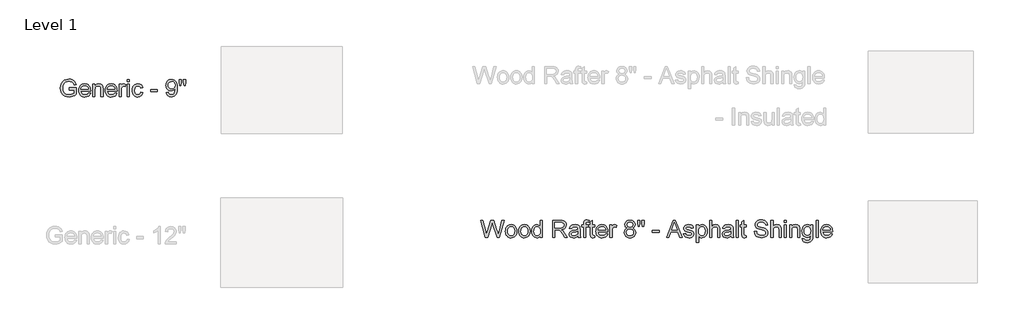
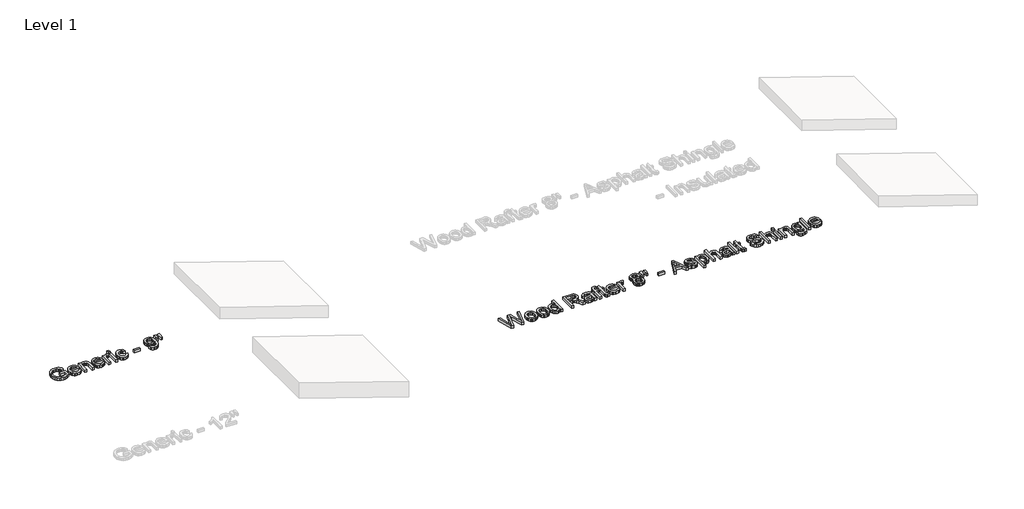
# One storey, part 7 of 42: 2 proxies.
"""IFC4 building model written with IfcOpenShell, lengths in millimetres."""

from ifc_helpers import new_model, si_unit, origin, origin_with_axes, place, context, project, spatial, polyline, outline, extrude, element, save

model = new_model("IFC4")

# Units and contexts
model_context = context("Model", 3, world=origin())
ifc_project = project(units=[si_unit("LENGTHUNIT", "METRE", prefix="MILLI")], contexts=[model_context])

# Site, building, storey
site = spatial("IfcSite", under=ifc_project)
building = spatial("IfcBuilding", under=site)
storey = spatial("IfcBuildingStorey", under=building, Name="Level 1", Elevation=0.0)

# Proxies
placement = place(None, origin())
element("IfcBuildingElementProxy", 1, Name="8\" Arial", ObjectType="8\" Arial", at=placement, inside=storey, context=model_context, shape_type="SweptSolid", body=[
    extrude(outline(polyline([(-15459.1576227, -5830.4947741), (-15459.1576227, -5792.4238873), (-15335.4272408, -5792.4238873), (-15335.4272408, -5906.2647616), (-15365.4954338, -5927.1777243), (-15396.5116812, -5942.1792895), (-15428.4016256, -5951.2136894), (-15461.09091, -5954.2251561), (-15503.7998271, -5949.4384113), (-15542.4005089, -5935.0781769), (-15574.4670517, -5911.646364), (-15597.5735518, -5879.6448838), (-15611.5434109, -5841.2579789), (-15616.2000306, -5798.6698922), (-15611.5620002, -5755.775082), (-15597.647909, -5715.8731492), (-15575.0340254, -5682.4031143), (-15560.680762, -5669.3696912), (-15544.2966175, -5658.8039977), (-15506.857767, -5644.8062546), (-15464.1395552, -5640.1403403), (-15432.7794058, -5642.8450835), (-15404.5794374, -5650.959313), (-15380.8316065, -5663.8974659), (-15362.8278692, -5681.0739793), (-15349.5086357, -5703.3160769), (-15339.8143156, -5731.4509828), (-15374.9109143, -5741.3404905), (-15382.7463044, -5721.2733409), (-15392.2733207, -5706.1323559), (-15404.8768662, -5694.7185256), (-15421.9418438, -5685.8328401), (-15442.2878328, -5680.1166303), (-15464.7344128, -5678.2112271), (-15491.0103886, -5680.2653447), (-15513.4755579, -5686.4276977), (-15532.0462687, -5695.9268301), (-15546.6388694, -5707.9912859), (-15566.2319917, -5737.3252016), (-15575.1548558, -5766.0642597), (-15578.1291439, -5797.108391), (-15574.5507036, -5833.5155354), (-15563.8153827, -5863.4721926), (-15546.2484941, -5886.7645857), (-15522.1753503, -5903.1789378), (-15494.0032659, -5912.9104364), (-15464.1395552, -5916.1542693), (-15437.7706329, -5913.7097763), (-15412.0523361, -5906.3762974), (-15389.7172919, -5896.2730128), (-15373.4981275, -5885.5191026), (-15373.4981275, -5830.4947741), (-15459.1576227, -5830.4947741)])), origin_with_axes(), (0.0, 0.0, 1.0), 50.8),
    extrude(outline(polyline([(-15121.724646, -5882.8422434), (-15084.3973312, -5887.6011042), (-15097.8466899, -5915.7267154), (-15119.3080369, -5936.7512139), (-15148.2980506, -5949.8566705), (-15184.333409, -5954.2251561), (-15207.9557621, -5952.3406658), (-15229.0034973, -5946.6871948), (-15247.4766143, -5937.2647433), (-15263.3751133, -5924.0733112), (-15276.1599045, -5907.4800371), (-15285.2918982, -5887.8520598), (-15290.7710944, -5865.1893792), (-15292.5974932, -5839.4919954), (-15290.7525051, -5812.9232381), (-15285.217541, -5789.5053672), (-15275.9926008, -5769.2383827), (-15263.0776845, -5752.1222846), (-15247.2210114, -5738.5242115), (-15229.170801, -5728.8113021), (-15208.9270531, -5722.9835565), (-15186.4897678, -5721.0409747), (-15164.7751415, -5722.9789092), (-15145.1378695, -5728.7927128), (-15127.5779519, -5738.4823856), (-15112.0953885, -5752.0479274), (-15099.456988, -5769.1268469), (-15090.4295591, -5789.3566528), (-15085.0131018, -5812.7373451), (-15083.207616, -5839.2689238), (-15083.4306876, -5849.5302175), (-15254.5266064, -5849.5302175), (-15247.9366995, -5878.0276146), (-15232.6284108, -5898.9777559), (-15210.5350275, -5911.860141), (-15183.5898369, -5916.1542693), (-15163.3274998, -5914.1652142), (-15146.2625222, -5908.1980488), (-15132.3949043, -5897.8809872), (-15121.724646, -5882.8422434)]), holes=[polyline([(-15254.5266064, -5811.4593307), (-15121.2785028, -5811.4593307), (-15126.4277389, -5791.3457079), (-15136.5217289, -5776.9575896), (-15158.7173533, -5763.5732935), (-15186.6384822, -5759.1118614), (-15212.3010111, -5762.6717124), (-15233.5206972, -5773.3512654), (-15248.2713069, -5789.9979837), (-15254.5266064, -5811.4593307)])]), origin_with_axes(), (0.0, 0.0, 1.0), 50.8),
    extrude(outline(polyline([(-15045.1367292, -5949.4662952), (-15045.1367292, -5725.7998355), (-15007.0658425, -5725.7998355), (-15007.0658425, -5757.0298598), (-14993.8395554, -5741.2847226), (-14977.9549984, -5730.0381959), (-14959.4121715, -5723.29028), (-14938.2110746, -5721.0409747), (-14919.4451761, -5722.8534314), (-14902.2593681, -5728.2908017), (-14887.9270177, -5736.6745761), (-14877.7214919, -5747.3262451), (-14866.3076616, -5775.3217312), (-14864.3000171, -5812.1285455), (-14864.3000171, -5949.4662952), (-14902.3709039, -5949.4662952), (-14902.3709039, -5817.2591924), (-14906.7579787, -5783.5753805), (-14912.8273852, -5773.546453), (-14922.2614551, -5765.7668309), (-14934.3537948, -5760.7756038), (-14948.3980111, -5759.1118614), (-14970.6958767, -5762.8483108), (-14989.7034361, -5774.0576588), (-14997.2994889, -5783.2082418), (-15002.7252409, -5795.7141935), (-15007.0658425, -5830.7922029), (-15007.0658425, -5949.4662952), (-15045.1367292, -5949.4662952)])), origin_with_axes(), (0.0, 0.0, 1.0), 50.8),
    extrude(outline(polyline([(-14655.3562832, -5882.8422434), (-14618.0289684, -5887.6011042), (-14631.4783271, -5915.7267154), (-14652.9396741, -5936.7512139), (-14681.9296878, -5949.8566705), (-14717.9650462, -5954.2251561), (-14741.5873994, -5952.3406658), (-14762.6351345, -5946.6871948), (-14781.1082515, -5937.2647433), (-14797.0067505, -5924.0733112), (-14809.7915417, -5907.4800371), (-14818.9235354, -5887.8520598), (-14824.4027316, -5865.1893792), (-14826.2291304, -5839.4919954), (-14824.3841423, -5812.9232381), (-14818.8491782, -5789.5053672), (-14809.624238, -5769.2383827), (-14796.7093217, -5752.1222846), (-14780.8526487, -5738.5242115), (-14762.8024382, -5728.8113021), (-14742.5586903, -5722.9835565), (-14720.121405, -5721.0409747), (-14698.4067787, -5722.9789092), (-14678.7695067, -5728.7927128), (-14661.2095891, -5738.4823856), (-14645.7270257, -5752.0479274), (-14633.0886252, -5769.1268469), (-14624.0611963, -5789.3566528), (-14618.644739, -5812.7373451), (-14616.8392532, -5839.2689238), (-14617.0623248, -5849.5302175), (-14788.1582436, -5849.5302175), (-14781.5683367, -5878.0276146), (-14766.260048, -5898.9777559), (-14744.1666648, -5911.860141), (-14717.2214742, -5916.1542693), (-14696.959137, -5914.1652142), (-14679.8941594, -5908.1980488), (-14666.0265415, -5897.8809872), (-14655.3562832, -5882.8422434)]), holes=[polyline([(-14788.1582436, -5811.4593307), (-14654.91014, -5811.4593307), (-14660.0593761, -5791.3457079), (-14670.1533661, -5776.9575896), (-14692.3489905, -5763.5732935), (-14720.2701194, -5759.1118614), (-14745.9326483, -5762.6717124), (-14767.1523344, -5773.3512654), (-14781.9029441, -5789.9979837), (-14788.1582436, -5811.4593307)])]), origin_with_axes(), (0.0, 0.0, 1.0), 50.8),
    extrude(outline(polyline([(-14578.7683664, -5949.4662952), (-14578.7683664, -5725.7998355), (-14545.4563405, -5725.7998355), (-14545.4563405, -5758.8887898), (-14533.1502238, -5739.704632), (-14521.8107507, -5728.4023375), (-14510.434099, -5722.8813154), (-14498.0164465, -5721.0409747), (-14479.0553603, -5723.9780841), (-14459.7968453, -5732.7894124), (-14472.5119266, -5766.9193675), (-14485.8962228, -5761.0637379), (-14499.2805189, -5759.1118614), (-14510.647876, -5760.9893807), (-14520.8069285, -5766.6219387), (-14529.0141045, -5775.5819814), (-14534.525832, -5787.4419549), (-14539.1545678, -5808.7081143), (-14540.6974797, -5831.9075609), (-14540.6974797, -5949.4662952), (-14578.7683664, -5949.4662952)])), origin_with_axes(), (0.0, 0.0, 1.0), 50.8),
    extrude(outline(polyline([(-14436.0025411, -5682.9700879), (-14436.0025411, -5644.8992011), (-14397.9316543, -5644.8992011), (-14397.9316543, -5682.9700879), (-14436.0025411, -5682.9700879)])), origin_with_axes(), (0.0, 0.0, 1.0), 50.8),
    extrude(outline(polyline([(-14436.0025411, -5949.4662952), (-14436.0025411, -5725.7998355), (-14397.9316543, -5725.7998355), (-14397.9316543, -5949.4662952), (-14436.0025411, -5949.4662952)])), origin_with_axes(), (0.0, 0.0, 1.0), 50.8),
    extrude(outline(polyline([(-14198.0594989, -5868.5656609), (-14159.9886121, -5873.3245217), (-14170.6031025, -5907.184932), (-14190.5494216, -5932.7731037), (-14217.9500501, -5948.862143), (-14250.9274686, -5954.2251561), (-14272.2796035, -5952.3546077), (-14291.424259, -5946.7429627), (-14308.3614351, -5937.3902211), (-14323.0911318, -5924.2963828), (-14335.0138442, -5907.707756), (-14343.5300674, -5887.8706491), (-14348.6398013, -5864.7850619), (-14350.3430459, -5838.4509946), (-14347.4338204, -5804.571995), (-14338.706144, -5775.2101954), (-14324.0205969, -5751.499543), (-14303.2377593, -5734.5739852), (-14278.3745703, -5724.4242273), (-14251.447969, -5721.0409747), (-14219.279185, -5725.6882997), (-14193.5608882, -5739.6302748), (-14175.1110078, -5762.1233281), (-14164.747473, -5792.4238873), (-14202.8183597, -5797.1827482), (-14209.7242847, -5780.5732085), (-14220.4781949, -5768.6667617), (-14234.4852326, -5761.5005865), (-14251.1505402, -5759.1118614), (-14275.7534789, -5763.8149544), (-14295.2815388, -5777.9242332), (-14308.024504, -5802.2018592), (-14312.2721591, -5837.4099938), (-14308.1174506, -5873.0921554), (-14295.6533248, -5897.4534333), (-14276.4784617, -5911.4790603), (-14252.191541, -5916.1542693), (-14232.4775881, -5913.2357492), (-14216.3141916, -5904.4801888), (-14204.5564593, -5889.6645166), (-14198.0594989, -5868.5656609)])), origin_with_axes(), (0.0, 0.0, 1.0), 50.8),
    extrude(outline(polyline([(-14026.7405085, -5859.0479392), (-14026.7405085, -5820.9770524), (-13907.7689873, -5820.9770524), (-13907.7689873, -5859.0479392), (-14026.7405085, -5859.0479392)])), origin_with_axes(), (0.0, 0.0, 1.0), 50.8),
    extrude(outline(polyline([(-13750.7265795, -5873.3245217), (-13712.6556927, -5868.5656609), (-13706.1494376, -5890.1757223), (-13695.5535365, -5904.8891534), (-13681.1282396, -5913.3379903), (-13663.133797, -5916.1542693), (-13646.9889898, -5914.3418125), (-13632.3127373, -5908.9044422), (-13620.1181564, -5900.437016), (-13611.4183639, -5889.5343915), (-13598.9635328, -5856.4454371), (-13593.4611, -5812.2772599), (-13593.6841716, -5804.8415399), (-13606.87328, -5820.9398738), (-13624.1334453, -5833.6921337), (-13644.2191841, -5842.0015509), (-13665.8850135, -5844.7713566), (-13683.9700789, -5843.0797303), (-13700.6005315, -5838.0048514), (-13715.7763715, -5829.5467198), (-13729.4975987, -5817.7053356), (-13740.8672794, -5803.098793), (-13748.9884799, -5786.3451862), (-13753.8612002, -5767.4445152), (-13755.4854403, -5746.3967801), (-13753.7821957, -5724.6472989), (-13748.6724618, -5705.1285337), (-13740.1562386, -5687.8404846), (-13728.2335262, -5672.7831514), (-13713.7454904, -5660.5839232), (-13697.533297, -5651.8701887), (-13679.596946, -5646.641948), (-13659.9364374, -5644.8992011), (-13631.5412814, -5648.8773114), (-13605.6928595, -5660.8116421), (-13584.0735034, -5680.1073357), (-13568.3655447, -5706.1695345), (-13558.8013498, -5742.1955983), (-13555.6132848, -5791.3828865), (-13558.7920551, -5843.5351682), (-13568.3283661, -5883.8460656), (-13584.1385659, -5914.1373302), (-13606.1390027, -5936.2307135), (-13633.3816221, -5949.7265454), (-13664.9183698, -5954.2251561), (-13697.4682344, -5948.9179109), (-13723.4374868, -5932.9961753), (-13741.5992331, -5907.4637715), (-13750.7265795, -5873.3245217)]), holes=[polyline([(-13593.6841716, -5745.5044937), (-13597.7924069, -5719.7025451), (-13610.1171129, -5699.8491725), (-13629.2455028, -5687.189859), (-13653.7647897, -5682.9700879), (-13679.1949524, -5687.5151718), (-13699.5688254, -5701.1504235), (-13712.9531215, -5722.0169129), (-13717.4145535, -5748.2557101), (-13713.1947824, -5771.7804695), (-13700.535469, -5790.4534215), (-13680.6635071, -5802.6387078), (-13654.8057905, -5806.7004699), (-13630.4816913, -5802.6387078), (-13610.8978635, -5790.4534215), (-13597.9875946, -5771.0926654), (-13593.6841716, -5745.5044937)])]), origin_with_axes(), (0.0, 0.0, 1.0), 50.8),
    extrude(outline(polyline([(-13513.0066088, -5754.3530006), (-13522.3012589, -5695.5364548), (-13522.3012589, -5644.8992011), (-13484.2303721, -5644.8992011), (-13484.2303721, -5695.5364548), (-13492.5583786, -5754.3530006), (-13513.0066088, -5754.3530006)])), origin_with_axes(), (0.0, 0.0, 1.0), 50.8),
    extrude(outline(polyline([(-13437.0879069, -5754.3530006), (-13446.1594854, -5695.5364548), (-13446.1594854, -5644.8992011), (-13408.0885986, -5644.8992011), (-13408.0885986, -5695.5364548), (-13417.0114627, -5754.3530006), (-13437.0879069, -5754.3530006)])), origin_with_axes(), (0.0, 0.0, 1.0), 50.8),
])
element("IfcBuildingElementProxy", 2, Name="8\" Arial", ObjectType="8\" Arial", at=placement, inside=storey, context=model_context, shape_type="SweptSolid", body=[
    extrude(outline(polyline([(-8126.3343653, -8434.4968379), (-8209.3913584, -8129.9297438), (-8170.1307565, -8129.9297438), (-8121.9472904, -8330.0993281), (-8107.0758503, -8391.8901619), (-8091.1634093, -8337.2376193), (-8030.7853624, -8129.9297438), (-7974.1995326, -8129.9297438), (-7930.3287842, -8280.2056464), (-7911.5350017, -8335.9735469), (-7897.6859731, -8391.8901619), (-7883.2606762, -8331.8839009), (-7834.6310669, -8129.9297438), (-7795.3704649, -8129.9297438), (-7878.5018153, -8434.4968379), (-7919.1752041, -8434.4968379), (-7992.1939752, -8199.5280836), (-8002.3809117, -8166.7365581), (-8013.8319206, -8206.2202317), (-8080.3816152, -8434.4968379), (-8126.3343653, -8434.4968379)])), origin_with_axes(), (0.0, 0.0, 1.0), 50.8),
    extrude(outline(polyline([(-7771.5761607, -8322.663608), (-7769.5173957, -8293.696831), (-7763.3411007, -8268.7360482), (-7753.0472758, -8247.7812596), (-7738.6359208, -8230.8324651), (-7724.126972, -8219.9995505), (-7708.1122899, -8212.2617543), (-7690.5918745, -8207.6190766), (-7671.5657258, -8206.0715173), (-7650.5621402, -8207.9560076), (-7631.5708464, -8213.6094785), (-7614.5918444, -8223.0319301), (-7599.6251341, -8236.2233622), (-7587.4096402, -8252.7376317), (-7578.6842874, -8272.1285955), (-7573.4490758, -8294.3962534), (-7571.7040052, -8319.5406056), (-7574.7898291, -8358.0018676), (-7584.0473005, -8387.2800154), (-7599.2068748, -8409.206095), (-7619.9990071, -8425.6111524), (-7644.6948924, -8435.8445621), (-7671.5657258, -8439.2556987), (-7692.8760348, -8437.3781794), (-7712.0439269, -8431.7456214), (-7729.0694022, -8422.3580248), (-7743.9524607, -8409.2153896), (-7756.0378294, -8392.5407874), (-7764.6702357, -8372.5572897), (-7769.8496795, -8349.2648966), (-7771.5761607, -8322.663608)]), holes=[polyline([(-7733.505274, -8322.5892508), (-7729.0996098, -8357.0445187), (-7715.8826174, -8381.5916896), (-7695.9920662, -8396.2865314), (-7671.5657258, -8401.1848119), (-7647.2509211, -8396.2586474), (-7627.3975486, -8381.4801538), (-7614.1805561, -8356.6076701), (-7609.774892, -8321.3995356), (-7614.2084401, -8287.9480899), (-7627.5090844, -8263.7355265), (-7647.3903409, -8249.0406847), (-7671.5657258, -8244.1424041), (-7695.9920662, -8249.0220954), (-7715.8826174, -8263.6611693), (-7729.0996098, -8288.1525722), (-7733.505274, -8322.5892508)])]), origin_with_axes(), (0.0, 0.0, 1.0), 50.8),
    extrude(outline(polyline([(-7538.3919793, -8322.663608), (-7536.3332143, -8293.696831), (-7530.1569193, -8268.7360482), (-7519.8630944, -8247.7812596), (-7505.4517394, -8230.8324651), (-7490.9427906, -8219.9995505), (-7474.9281085, -8212.2617543), (-7457.4076931, -8207.6190766), (-7438.3815444, -8206.0715173), (-7417.3779588, -8207.9560076), (-7398.386665, -8213.6094785), (-7381.407663, -8223.0319301), (-7366.4409527, -8236.2233622), (-7354.2254588, -8252.7376317), (-7345.5001061, -8272.1285955), (-7340.2648944, -8294.3962534), (-7338.5198238, -8319.5406056), (-7341.6056477, -8358.0018676), (-7350.8631192, -8387.2800154), (-7366.0226934, -8409.206095), (-7386.8148257, -8425.6111524), (-7411.510711, -8435.8445621), (-7438.3815444, -8439.2556987), (-7459.6918534, -8437.3781794), (-7478.8597455, -8431.7456214), (-7495.8852208, -8422.3580248), (-7510.7682793, -8409.2153896), (-7522.853648, -8392.5407874), (-7531.4860543, -8372.5572897), (-7536.6654981, -8349.2648966), (-7538.3919793, -8322.663608)]), holes=[polyline([(-7500.3210926, -8322.5892508), (-7495.9154284, -8357.0445187), (-7482.698436, -8381.5916896), (-7462.8078848, -8396.2865314), (-7438.3815444, -8401.1848119), (-7414.0667397, -8396.2586474), (-7394.2133672, -8381.4801538), (-7380.9963747, -8356.6076701), (-7376.5907106, -8321.3995356), (-7381.0242587, -8287.9480899), (-7394.324903, -8263.7355265), (-7414.2061595, -8249.0406847), (-7438.3815444, -8244.1424041), (-7462.8078848, -8249.0220954), (-7482.698436, -8263.6611693), (-7495.9154284, -8288.1525722), (-7500.3210926, -8322.5892508)])]), origin_with_axes(), (0.0, 0.0, 1.0), 50.8),
    extrude(outline(polyline([(-7157.6831117, -8434.4968379), (-7157.6831117, -8398.5823099), (-7169.0737054, -8416.3769175), (-7182.8716135, -8429.0873515), (-7199.0768359, -8436.7136119), (-7217.6893727, -8439.2556987), (-7242.3016061, -8435.5750173), (-7264.8318379, -8424.532973), (-7283.9044599, -8406.9010218), (-7298.1438639, -8383.4506196), (-7307.01096, -8355.1298208), (-7309.9666588, -8322.8866796), (-7307.2433263, -8291.0432084), (-7299.0733289, -8262.285561), (-7285.4659611, -8238.2495959), (-7266.4305178, -8220.5711714), (-7243.4076695, -8209.6964308), (-7217.8380871, -8206.0715173), (-7199.2116083, -8208.6647247), (-7182.7414884, -8216.4443468), (-7168.7809239, -8228.3693829), (-7157.6831117, -8243.3988321), (-7157.6831117, -8129.9297438), (-7119.612225, -8129.9297438), (-7119.612225, -8434.4968379), (-7157.6831117, -8434.4968379)]), holes=[polyline([(-7271.895772, -8322.7379652), (-7267.6016437, -8357.1746438), (-7254.7192586, -8381.6660468), (-7235.9998334, -8396.3051207), (-7214.1945843, -8401.1848119), (-7192.3986298, -8396.5281923), (-7174.1532317, -8382.5583332), (-7161.8006417, -8359.0149845), (-7157.6831117, -8325.637896), (-7161.8749989, -8289.1470998), (-7174.4506605, -8263.8470623), (-7193.1607911, -8249.0685686), (-7215.7560855, -8244.1424041), (-7237.7844062, -8248.873381), (-7255.8346167, -8263.0663116), (-7267.8804832, -8287.4461788), (-7271.895772, -8322.7379652)])]), origin_with_axes(), (0.0, 0.0, 1.0), 50.8),
    extrude(outline(polyline([(-6938.7755129, -8434.4968379), (-6938.7755129, -8129.9297438), (-6807.5350536, -8129.9297438), (-6772.2618566, -8131.9838615), (-6746.5993277, -8138.1462145), (-6727.8427238, -8149.5228662), (-6713.2873017, -8167.2198799), (-6703.9461784, -8189.1645488), (-6700.8324706, -8213.2841658), (-6705.9910014, -8243.2872963), (-6721.4665938, -8268.1597799), (-6733.1894712, -8278.2955958), (-6747.7239803, -8286.3958834), (-6785.2278934, -8296.4898734), (-6763.589948, -8312.7741003), (-6732.7317097, -8351.9603451), (-6681.9457417, -8434.4968379), (-6726.1882761, -8434.4968379), (-6765.820664, -8371.3675745), (-6794.4481863, -8329.5788277), (-6814.5618091, -8309.8369909), (-6832.6677875, -8302.5871638), (-6854.7518761, -8301.2487342), (-6900.7046261, -8301.2487342), (-6900.7046261, -8434.4968379), (-6938.7755129, -8434.4968379)]), holes=[polyline([(-6900.7046261, -8263.1778474), (-6815.4912741, -8263.1778474), (-6791.0184604, -8261.8301232), (-6772.0294903, -8257.7869504), (-6757.7343185, -8250.7787842), (-6747.3428997, -8240.5360798), (-6741.013243, -8228.1463113), (-6738.9033574, -8214.6969526), (-6742.9279409, -8196.1262417), (-6755.0016913, -8181.1618551), (-6775.7752343, -8171.2909367), (-6805.8991952, -8168.0006306), (-6900.7046261, -8168.0006306), (-6900.7046261, -8263.1778474)])]), origin_with_axes(), (0.0, 0.0, 1.0), 50.8),
    extrude(outline(polyline([(-6496.2014543, -8405.9436728), (-6514.3910845, -8421.5400956), (-6533.1198044, -8431.7456214), (-6552.815168, -8437.3781794), (-6573.904729, -8439.2556987), (-6605.7203163, -8434.7384988), (-6629.1893078, -8421.1868989), (-6643.6610779, -8400.6085436), (-6648.4850013, -8375.0110773), (-6646.6632499, -8359.2287615), (-6641.1979957, -8344.896411), (-6632.767748, -8332.6274729), (-6622.0510165, -8323.035394), (-6595.39396, -8310.5433843), (-6562.4537201, -8304.8178798), (-6523.5277256, -8298.7949466), (-6496.4245259, -8291.7310125), (-6496.2014543, -8283.2542916), (-6498.8225456, -8266.2636713), (-6506.6858196, -8255.1472698), (-6524.2712976, -8246.8936205), (-6548.7719952, -8244.1424041), (-6571.4509414, -8245.9734501), (-6587.2890252, -8251.4665883), (-6598.0894086, -8261.6256409), (-6605.6552537, -8277.45443), (-6643.7261405, -8272.6955691), (-6637.1176443, -8251.8755529), (-6627.2560205, -8235.5169688), (-6613.2210989, -8223.0063698), (-6594.092709, -8213.730309), (-6570.6980748, -8207.9862152), (-6543.86442, -8206.0715173), (-6518.1275339, -8207.7631436), (-6497.7257769, -8212.8380226), (-6482.343131, -8220.4689303), (-6471.6635781, -8229.8286429), (-6464.5810547, -8241.4004823), (-6459.9894976, -8255.6677702), (-6458.1305675, -8288.9797961), (-6458.1305675, -8336.3453329), (-6456.1972803, -8402.486063), (-6448.6128459, -8434.4968379), (-6486.6837326, -8434.4968379), (-6492.7810231, -8421.2612561), (-6496.2014543, -8405.9436728)]), holes=[polyline([(-6496.2014543, -8329.8018993), (-6557.6205021, -8341.4759798), (-6590.374849, -8347.6476274), (-6605.2091105, -8357.6858495), (-6610.4141146, -8372.3342181), (-6607.5792463, -8383.6551019), (-6599.0746415, -8392.9311627), (-6585.0861931, -8399.1213996), (-6565.7997942, -8401.1848119), (-6545.351564, -8398.9076227), (-6527.2827642, -8392.0760549), (-6512.6343957, -8382.0099488), (-6502.4474592, -8370.0291449), (-6497.9302592, -8357.6858495), (-6496.4245259, -8340.5836934), (-6496.2014543, -8329.8018993)])]), origin_with_axes(), (0.0, 0.0, 1.0), 50.8),
    extrude(outline(polyline([(-6396.2653766, -8434.4968379), (-6396.2653766, -8248.9012649), (-6429.5774025, -8248.9012649), (-6429.5774025, -8210.8303782), (-6396.2653766, -8210.8303782), (-6396.2653766, -8188.3001463), (-6392.2500877, -8156.5496216), (-6384.5912961, -8143.8903082), (-6372.7685011, -8133.8706754), (-6356.224024, -8127.3458311), (-6334.4001856, -8125.1708829), (-6299.6753729, -8129.3348862), (-6305.2521629, -8165.0263425), (-6327.1875371, -8163.2417697), (-6341.6593073, -8164.8218602), (-6351.1677343, -8169.5621318), (-6356.4378009, -8178.615121), (-6358.1944898, -8193.1333644), (-6358.1944898, -8210.8303782), (-6315.3647422, -8210.8303782), (-6315.3647422, -8248.9012649), (-6358.1944898, -8248.9012649), (-6358.1944898, -8434.4968379), (-6396.2653766, -8434.4968379)])), origin_with_axes(), (0.0, 0.0, 1.0), 50.8),
    extrude(outline(polyline([(-6201.1520819, -8402.7463132), (-6196.3932211, -8435.6121959), (-6224.8720289, -8439.2556987), (-6243.145311, -8437.6756082), (-6256.771268, -8432.9353366), (-6266.4005255, -8425.6297417), (-6272.683709, -8416.3536809), (-6276.1413188, -8400.4226506), (-6277.2938554, -8373.1521473), (-6277.2938554, -8248.9012649), (-6305.8470205, -8248.9012649), (-6305.8470205, -8210.8303782), (-6277.2938554, -8210.8303782), (-6277.2938554, -8156.4752644), (-6239.2229687, -8134.093747), (-6239.2229687, -8210.8303782), (-6201.1520819, -8210.8303782), (-6201.1520819, -8248.9012649), (-6239.2229687, -8248.9012649), (-6239.2229687, -8372.0367893), (-6237.2153243, -8391.6670903), (-6230.7090692, -8398.6194885), (-6217.7337377, -8401.1848119), (-6201.1520819, -8402.7463132)])), origin_with_axes(), (0.0, 0.0, 1.0), 50.8),
    extrude(outline(polyline([(-6006.4849305, -8367.872786), (-5969.1576157, -8372.6316469), (-5982.6069744, -8400.757258), (-6004.0683215, -8421.7817565), (-6033.0583351, -8434.8872132), (-6069.0936935, -8439.2556987), (-6092.7160467, -8437.3712084), (-6113.7637818, -8431.7177375), (-6132.2368988, -8422.295286), (-6148.1353978, -8409.1038538), (-6160.920189, -8392.5105798), (-6170.0521827, -8372.8826024), (-6175.531379, -8350.2199219), (-6177.3577777, -8324.522538), (-6175.5127897, -8297.9537808), (-6169.9778255, -8274.5359099), (-6160.7528853, -8254.2689253), (-6147.837969, -8237.1528272), (-6131.981296, -8223.5547541), (-6113.9310855, -8213.8418448), (-6093.6873376, -8208.0140992), (-6071.2500523, -8206.0715173), (-6049.535426, -8208.0094519), (-6029.8981541, -8213.8232555), (-6012.3382364, -8223.5129282), (-5996.855673, -8237.07847), (-5984.2172725, -8254.1573895), (-5975.1898436, -8274.3871955), (-5969.7733863, -8297.7678877), (-5967.9679005, -8324.2994664), (-5968.1909721, -8334.5607601), (-6139.2868909, -8334.5607601), (-6132.696984, -8363.0581573), (-6117.3886953, -8384.0082986), (-6095.2953121, -8396.8906836), (-6068.3501215, -8401.1848119), (-6048.0877843, -8399.1957568), (-6031.0228067, -8393.2285915), (-6017.1551888, -8382.9115299), (-6006.4849305, -8367.872786)]), holes=[polyline([(-6139.2868909, -8296.4898734), (-6006.0387873, -8296.4898734), (-6011.1880234, -8276.3762506), (-6021.2820134, -8261.9881322), (-6043.4776378, -8248.6038361), (-6071.3987667, -8244.1424041), (-6097.0612956, -8247.7022551), (-6118.2809817, -8258.381808), (-6133.0315914, -8275.0285263), (-6139.2868909, -8296.4898734)])]), origin_with_axes(), (0.0, 0.0, 1.0), 50.8),
    extrude(outline(polyline([(-5929.8970138, -8434.4968379), (-5929.8970138, -8210.8303782), (-5896.5849879, -8210.8303782), (-5896.5849879, -8243.9193325), (-5884.2788711, -8224.7351747), (-5872.939398, -8213.4328802), (-5861.5627463, -8207.911858), (-5849.1450938, -8206.0715173), (-5830.1840076, -8209.0086267), (-5810.9254926, -8217.819955), (-5823.640574, -8251.9499101), (-5837.0248701, -8246.0942806), (-5850.4091662, -8244.1424041), (-5861.7765233, -8246.0199234), (-5871.9355758, -8251.6524813), (-5880.1427518, -8260.612524), (-5885.6544794, -8272.4724975), (-5890.2832151, -8293.7386569), (-5891.826127, -8316.9381036), (-5891.826127, -8434.4968379), (-5929.8970138, -8434.4968379)])), origin_with_axes(), (0.0, 0.0, 1.0), 50.8),
    extrude(outline(polyline([(-5622.2069173, -8266.7469931), (-5642.5900849, -8256.708771), (-5656.8945514, -8243.1014033), (-5665.3433883, -8226.2037294), (-5668.1596673, -8206.2945889), (-5666.62605, -8190.7678759), (-5662.0251982, -8176.5331193), (-5654.3571119, -8163.5903191), (-5643.6217911, -8151.9394752), (-5630.3350888, -8142.3102177), (-5615.0128581, -8135.4321766), (-5578.2618117, -8129.9297438), (-5541.2876936, -8135.5623017), (-5525.7981592, -8142.6029992), (-5512.3069746, -8152.4599756), (-5501.3764661, -8164.3385384), (-5493.5689601, -8177.443995), (-5488.8844564, -8191.7763455), (-5487.3229552, -8207.3355897), (-5490.1020556, -8226.6033994), (-5498.4393567, -8243.2129391), (-5512.4278051, -8256.7366549), (-5532.1603472, -8266.7469931), (-5508.7285344, -8278.8207435), (-5491.6728514, -8296.6014092), (-5481.272138, -8319.2338821), (-5477.8052335, -8345.8630546), (-5479.5247438, -8364.8520248), (-5484.6832746, -8382.2609044), (-5493.2808259, -8398.0896935), (-5505.3173978, -8412.3383921), (-5520.160954, -8424.1147137), (-5537.1794583, -8432.526372), (-5556.3729107, -8437.573367), (-5577.7413113, -8439.2556987), (-5599.1097118, -8437.5663961), (-5618.3031642, -8432.4984881), (-5635.3216685, -8424.0519748), (-5650.1652247, -8412.2268563), (-5662.2017966, -8397.8782402), (-5670.7993479, -8381.8612344), (-5675.9578787, -8364.175839), (-5677.677389, -8344.8220538), (-5674.0710648, -8317.1611752), (-5663.2520921, -8294.4078717), (-5645.7781499, -8277.3428942), (-5622.2069173, -8266.7469931)]), holes=[polyline([(-5630.0887805, -8207.4099469), (-5626.7148226, -8224.0287813), (-5616.5929486, -8237.3015416), (-5600.0205875, -8246.0013341), (-5577.295168, -8248.9012649), (-5555.0995436, -8246.0199234), (-5538.7781381, -8237.3758988), (-5528.739916, -8224.5492817), (-5525.393842, -8209.1201625), (-5528.8514518, -8193.1054804), (-5539.2242813, -8179.8606041), (-5555.7687584, -8170.9656239), (-5577.7413113, -8168.0006306), (-5599.8532838, -8170.9005614), (-5616.369877, -8179.6003539), (-5626.6590547, -8192.3526138), (-5630.0887805, -8207.4099469)]), polyline([(-5639.6065022, -8343.4836242), (-5638.0171171, -8358.0483409), (-5633.2489616, -8372.1483251), (-5624.4469279, -8384.4451471), (-5610.7559084, -8393.6003775), (-5594.3601456, -8399.2887033), (-5577.4438824, -8401.1848119), (-5551.530398, -8397.1974071), (-5532.08599, -8385.2351924), (-5519.9285877, -8367.1199194), (-5515.8761203, -8344.6733394), (-5520.0587128, -8321.8456788), (-5532.6064904, -8303.3307358), (-5552.4970416, -8291.0617977), (-5578.7079549, -8286.9721517), (-5604.258948, -8291.0060298), (-5623.5081683, -8303.1076642), (-5635.5819187, -8321.2694105), (-5639.6065022, -8343.4836242)])]), origin_with_axes(), (0.0, 0.0, 1.0), 50.8),
    extrude(outline(polyline([(-5435.1985575, -8239.3835432), (-5444.4932076, -8180.5669975), (-5444.4932076, -8129.9297438), (-5406.4223208, -8129.9297438), (-5406.4223208, -8180.5669975), (-5414.7503273, -8239.3835432), (-5435.1985575, -8239.3835432)])), origin_with_axes(), (0.0, 0.0, 1.0), 50.8),
    extrude(outline(polyline([(-5359.2798556, -8239.3835432), (-5368.3514341, -8180.5669975), (-5368.3514341, -8129.9297438), (-5330.2805473, -8129.9297438), (-5330.2805473, -8180.5669975), (-5339.2034114, -8239.3835432), (-5359.2798556, -8239.3835432)])), origin_with_axes(), (0.0, 0.0, 1.0), 50.8),
    extrude(outline(polyline([(-5182.7558611, -8344.0784818), (-5182.7558611, -8306.0075951), (-5063.78434, -8306.0075951), (-5063.78434, -8344.0784818), (-5182.7558611, -8344.0784818)])), origin_with_axes(), (0.0, 0.0, 1.0), 50.8),
    extrude(outline(polyline([(-4932.6925952, -8434.4968379), (-4811.118572, -8129.9297438), (-4778.6988325, -8129.9297438), (-4657.1248094, -8434.4968379), (-4697.352055, -8434.4968379), (-4732.2255821, -8339.319621), (-4857.6661797, -8339.319621), (-4892.4653496, -8434.4968379), (-4932.6925952, -8434.4968379)]), holes=[polyline([(-4843.6870259, -8301.2487342), (-4746.1303786, -8301.2487342), (-4773.5681857, -8226.3710331), (-4794.9087023, -8168.0006306), (-4813.8697885, -8219.8275994), (-4843.6870259, -8301.2487342)])]), origin_with_axes(), (0.0, 0.0, 1.0), 50.8),
    extrude(outline(polyline([(-4635.486864, -8367.872786), (-4597.4159772, -8363.1139252), (-4591.4116333, -8379.3981521), (-4579.7933207, -8391.3696615), (-4562.4866822, -8398.7310243), (-4539.4173607, -8401.1848119), (-4516.6268787, -8398.9355066), (-4500.6029019, -8392.1875907), (-4491.1223588, -8382.4096188), (-4487.9621778, -8371.0701457), (-4491.1409481, -8361.366531), (-4500.6772591, -8353.9679895), (-4539.8635039, -8343.1118382), (-4597.1929056, -8324.4853594), (-4611.7018544, -8315.1256468), (-4622.2141037, -8302.7358782), (-4628.5995283, -8288.106099), (-4630.7280031, -8272.0263543), (-4629.0177875, -8257.2757446), (-4623.8871407, -8243.6590823), (-4615.8007951, -8231.7154569), (-4605.2234833, -8221.9839583), (-4581.0202145, -8210.7188424), (-4548.2658676, -8206.0715173), (-4523.4863304, -8207.939742), (-4501.9413315, -8213.544416), (-4484.6161038, -8222.337155), (-4472.49588, -8233.7695746), (-4464.4653024, -8248.687488), (-4459.4090127, -8267.9367083), (-4497.4798995, -8272.6955691), (-4502.2852336, -8260.7147652), (-4511.7936606, -8251.6896599), (-4526.0981271, -8246.029218), (-4545.2915795, -8244.1424041), (-4567.1525965, -8245.9455662), (-4581.7266079, -8251.3550525), (-4589.9244892, -8259.1625586), (-4592.6571164, -8268.1597799), (-4588.1213271, -8279.2390028), (-4573.9191018, -8287.6413665), (-4541.1275763, -8295.7463014), (-4485.24814, -8313.6663867), (-4470.4882356, -8322.2360541), (-4459.2974769, -8333.9659025), (-4452.2428375, -8348.8931106), (-4449.891291, -8367.0548568), (-4452.6518021, -8385.83005), (-4460.9333353, -8403.4898852), (-4474.4198726, -8418.6494595), (-4492.7953958, -8429.92387), (-4514.9910202, -8436.9227415), (-4539.9378611, -8439.2556987), (-4578.3247659, -8434.7570881), (-4606.3388413, -8421.2612561), (-4625.0396773, -8398.9169173), (-4635.486864, -8367.872786)])), origin_with_axes(), (0.0, 0.0, 1.0), 50.8),
    extrude(outline(polyline([(-4407.0615434, -8520.1563331), (-4407.0615434, -8210.8303782), (-4368.9906567, -8210.8303782), (-4368.9906567, -8248.1576929), (-4356.5730042, -8229.7449911), (-4342.6682076, -8216.5930612), (-4326.4583379, -8208.7019033), (-4307.1254657, -8206.0715173), (-4281.3792849, -8209.7521987), (-4258.8676424, -8220.794243), (-4240.5385925, -8238.5284354), (-4227.3401893, -8262.285561), (-4219.3653796, -8290.336815), (-4216.7071096, -8320.9533924), (-4219.7092816, -8353.5125516), (-4228.7157975, -8382.6326904), (-4243.4385233, -8406.8359592), (-4263.5893247, -8424.6445088), (-4287.0583161, -8435.6029012), (-4311.7356121, -8439.2556987), (-4329.2374382, -8436.8112057), (-4344.861745, -8429.4777268), (-4358.2367465, -8418.4077986), (-4368.9906567, -8404.7539576), (-4368.9906567, -8520.1563331), (-4407.0615434, -8520.1563331)]), holes=[polyline([(-4368.9906567, -8324.4481808), (-4364.8731267, -8358.5781359), (-4352.5205367, -8382.4467974), (-4334.2937279, -8396.5003083), (-4312.5535413, -8401.1848119), (-4290.4601581, -8396.3330046), (-4271.7686168, -8381.7775826), (-4259.0256515, -8357.035224), (-4254.7779964, -8321.6226072), (-4258.9234103, -8287.6785451), (-4271.3596521, -8263.4752763), (-4289.558577, -8248.9756221), (-4310.9920401, -8244.1424041), (-4332.5091551, -8249.2823456), (-4351.4051787, -8264.7021701), (-4364.5942872, -8289.9185558), (-4368.9906567, -8324.4481808)])]), origin_with_axes(), (0.0, 0.0, 1.0), 50.8),
    extrude(outline(polyline([(-4173.877362, -8434.4968379), (-4173.877362, -8129.9297438), (-4135.8064753, -8129.9297438), (-4135.8064753, -8241.911688), (-4121.8226742, -8226.2316134), (-4106.1193629, -8215.03156), (-4088.6965413, -8208.311528), (-4069.5542094, -8206.0715173), (-4046.5592451, -8208.5160103), (-4026.798819, -8215.8494892), (-4011.2395748, -8227.4956858), (-4000.848156, -8242.8783317), (-3994.9925264, -8264.014366), (-3993.0406499, -8292.9207277), (-3993.0406499, -8434.4968379), (-4031.1115367, -8434.4968379), (-4031.1115367, -8296.8616594), (-4034.1415926, -8273.0301765), (-4043.2317604, -8256.708771), (-4057.8801289, -8247.2839958), (-4077.5847871, -8244.1424041), (-4093.6738264, -8246.2615843), (-4108.7776328, -8252.6191249), (-4121.2882318, -8262.6015791), (-4129.597649, -8275.5955), (-4134.2542687, -8292.8649598), (-4135.8064753, -8315.6740311), (-4135.8064753, -8434.4968379), (-4173.877362, -8434.4968379)])), origin_with_axes(), (0.0, 0.0, 1.0), 50.8),
    extrude(outline(polyline([(-3797.9273553, -8405.9436728), (-3816.1169855, -8421.5400956), (-3834.8457054, -8431.7456214), (-3854.541069, -8437.3781794), (-3875.63063, -8439.2556987), (-3907.4462173, -8434.7384988), (-3930.9152087, -8421.1868989), (-3945.3869789, -8400.6085436), (-3950.2109023, -8375.0110773), (-3948.3891509, -8359.2287615), (-3942.9238967, -8344.896411), (-3934.493649, -8332.6274729), (-3923.7769175, -8323.035394), (-3897.119861, -8310.5433843), (-3864.1796211, -8304.8178798), (-3825.2536265, -8298.7949466), (-3798.1504269, -8291.7310125), (-3797.9273553, -8283.2542916), (-3800.5484466, -8266.2636713), (-3808.4117206, -8255.1472698), (-3825.9971986, -8246.8936205), (-3850.4978962, -8244.1424041), (-3873.1768424, -8245.9734501), (-3889.0149261, -8251.4665883), (-3899.8153095, -8261.6256409), (-3907.3811547, -8277.45443), (-3945.4520415, -8272.6955691), (-3938.8435453, -8251.8755529), (-3928.9819215, -8235.5169688), (-3914.9469999, -8223.0063698), (-3895.81861, -8213.730309), (-3872.4239757, -8207.9862152), (-3845.5903209, -8206.0715173), (-3819.8534348, -8207.7631436), (-3799.4516779, -8212.8380226), (-3784.069032, -8220.4689303), (-3773.3894791, -8229.8286429), (-3766.3069557, -8241.4004823), (-3761.7153985, -8255.6677702), (-3759.8564685, -8288.9797961), (-3759.8564685, -8336.3453329), (-3757.9231813, -8402.486063), (-3750.3387468, -8434.4968379), (-3788.4096336, -8434.4968379), (-3794.5069241, -8421.2612561), (-3797.9273553, -8405.9436728)]), holes=[polyline([(-3797.9273553, -8329.8018993), (-3859.3464031, -8341.4759798), (-3892.10075, -8347.6476274), (-3906.9350115, -8357.6858495), (-3912.1400156, -8372.3342181), (-3909.3051473, -8383.6551019), (-3900.8005425, -8392.9311627), (-3886.8120941, -8399.1213996), (-3867.5256951, -8401.1848119), (-3847.077465, -8398.9076227), (-3829.0086652, -8392.0760549), (-3814.3602966, -8382.0099488), (-3804.1733601, -8370.0291449), (-3799.6561602, -8357.6858495), (-3798.1504269, -8340.5836934), (-3797.9273553, -8329.8018993)])]), origin_with_axes(), (0.0, 0.0, 1.0), 50.8),
    extrude(outline(polyline([(-3707.5089992, -8434.4968379), (-3707.5089992, -8129.9297438), (-3669.4381125, -8129.9297438), (-3669.4381125, -8434.4968379), (-3707.5089992, -8434.4968379)])), origin_with_axes(), (0.0, 0.0, 1.0), 50.8),
    extrude(outline(polyline([(-3531.431148, -8402.7463132), (-3526.6722871, -8435.6121959), (-3555.151095, -8439.2556987), (-3573.4243771, -8437.6756082), (-3587.0503341, -8432.9353366), (-3596.6795916, -8425.6297417), (-3602.9627751, -8416.3536809), (-3606.4203849, -8400.4226506), (-3607.5729215, -8373.1521473), (-3607.5729215, -8248.9012649), (-3636.1260866, -8248.9012649), (-3636.1260866, -8210.8303782), (-3607.5729215, -8210.8303782), (-3607.5729215, -8156.4752644), (-3569.5020347, -8134.093747), (-3569.5020347, -8210.8303782), (-3531.431148, -8210.8303782), (-3531.431148, -8248.9012649), (-3569.5020347, -8248.9012649), (-3569.5020347, -8372.0367893), (-3567.4943903, -8391.6670903), (-3560.9881353, -8398.6194885), (-3548.0128037, -8401.1848119), (-3531.431148, -8402.7463132)])), origin_with_axes(), (0.0, 0.0, 1.0), 50.8),
    extrude(outline(polyline([(-3383.9064618, -8329.8018993), (-3345.835575, -8329.8018993), (-3341.4670895, -8350.9286389), (-3333.5666369, -8367.9099646), (-3321.2419309, -8381.3872073), (-3303.600685, -8392.0016977), (-3282.0370968, -8398.8890334), (-3257.9453638, -8401.1848119), (-3236.7349723, -8399.4467124), (-3218.1642614, -8394.2324137), (-3203.1162229, -8385.9787644), (-3192.4738486, -8375.1226131), (-3186.1441919, -8362.6584873), (-3184.0343063, -8349.5809147), (-3185.6143968, -8336.8379494), (-3190.3546684, -8325.823789), (-3199.9839259, -8316.4268978), (-3216.2309742, -8308.5357399), (-3271.6642673, -8293.9989071), (-3308.0528224, -8284.3789443), (-3331.3359209, -8275.223714), (-3350.2877124, -8262.4156861), (-3363.7184818, -8246.8936205), (-3371.7211755, -8228.9921244), (-3374.3887401, -8209.0458053), (-3371.0891393, -8186.7479398), (-3361.190337, -8165.9558075), (-3344.9525833, -8148.333151), (-3322.6361284, -8135.5437124), (-3295.8489469, -8127.7640903), (-3266.1990131, -8125.1708829), (-3234.0767024, -8127.8849208), (-3205.9696805, -8136.0270343), (-3182.8817697, -8149.4299197), (-3165.8167921, -8167.9262734), (-3155.0164087, -8190.3635587), (-3150.7222804, -8215.589239), (-3188.7931672, -8215.589239), (-3195.782744, -8192.8731142), (-3210.3567554, -8176.4773514), (-3233.1286481, -8166.5506651), (-3264.7118691, -8163.2417697), (-3297.0386621, -8166.5134865), (-3319.2156972, -8176.328637), (-3332.0423143, -8190.7725233), (-3336.3178533, -8207.9304473), (-3333.2877974, -8222.5602266), (-3324.1976296, -8234.3272536), (-3302.7083986, -8244.8487975), (-3262.0350098, -8255.593413), (-3220.06037, -8265.7989388), (-3194.667386, -8274.7032136), (-3172.9643781, -8288.5150636), (-3157.8233931, -8305.5614518), (-3148.9284129, -8325.6564853), (-3145.9634196, -8348.6142711), (-3149.3745561, -8372.0832625), (-3159.6079659, -8394.1580565), (-3176.2453895, -8413.1563213), (-3198.8685678, -8427.3957252), (-3226.0740087, -8436.2907053), (-3256.4582198, -8439.2556987), (-3293.7576506, -8436.0583391), (-3324.4578798, -8426.4662602), (-3348.9121042, -8410.4422834), (-3367.4735204, -8387.9492302), (-3379.3892618, -8360.5486018), (-3383.9064618, -8329.8018993)])), origin_with_axes(), (0.0, 0.0, 1.0), 50.8),
    extrude(outline(polyline([(-3093.6159503, -8434.4968379), (-3093.6159503, -8129.9297438), (-3055.5450635, -8129.9297438), (-3055.5450635, -8241.911688), (-3041.5612624, -8226.2316134), (-3025.8579511, -8215.03156), (-3008.4351295, -8208.311528), (-2989.2927977, -8206.0715173), (-2966.2978334, -8208.5160103), (-2946.5374073, -8215.8494892), (-2930.978163, -8227.4956858), (-2920.5867442, -8242.8783317), (-2914.7311147, -8264.014366), (-2912.7792382, -8292.9207277), (-2912.7792382, -8434.4968379), (-2950.8501249, -8434.4968379), (-2950.8501249, -8296.8616594), (-2953.8801808, -8273.0301765), (-2962.9703486, -8256.708771), (-2977.6187172, -8247.2839958), (-2997.3233754, -8244.1424041), (-3013.4124147, -8246.2615843), (-3028.516221, -8252.6191249), (-3041.0268201, -8262.6015791), (-3049.3362372, -8275.5955), (-3053.9928569, -8292.8649598), (-3055.5450635, -8315.6740311), (-3055.5450635, -8434.4968379), (-3093.6159503, -8434.4968379)])), origin_with_axes(), (0.0, 0.0, 1.0), 50.8),
    extrude(outline(polyline([(-2860.4317689, -8168.0006306), (-2860.4317689, -8129.9297438), (-2822.3608821, -8129.9297438), (-2822.3608821, -8168.0006306), (-2860.4317689, -8168.0006306)])), origin_with_axes(), (0.0, 0.0, 1.0), 50.8),
    extrude(outline(polyline([(-2860.4317689, -8434.4968379), (-2860.4317689, -8210.8303782), (-2822.3608821, -8210.8303782), (-2822.3608821, -8434.4968379), (-2860.4317689, -8434.4968379)])), origin_with_axes(), (0.0, 0.0, 1.0), 50.8),
    extrude(outline(polyline([(-2765.254552, -8434.4968379), (-2765.254552, -8210.8303782), (-2727.1836652, -8210.8303782), (-2727.1836652, -8242.0604024), (-2713.9573781, -8226.3152652), (-2698.0728211, -8215.0687386), (-2679.5299942, -8208.3208226), (-2658.3288974, -8206.0715173), (-2639.5629988, -8207.8839741), (-2622.3771908, -8213.3213444), (-2608.0448404, -8221.7051188), (-2597.8393146, -8232.3567878), (-2586.4254843, -8260.3522738), (-2584.4178399, -8297.1590882), (-2584.4178399, -8434.4968379), (-2622.4887266, -8434.4968379), (-2622.4887266, -8302.289735), (-2626.8758015, -8268.6059231), (-2632.945208, -8258.5769957), (-2642.3792778, -8250.7973735), (-2654.4716176, -8245.8061464), (-2668.5158339, -8244.1424041), (-2690.8136994, -8247.8788534), (-2709.8212588, -8259.0882014), (-2717.4173116, -8268.2387844), (-2722.8430636, -8280.7447361), (-2727.1836652, -8315.8227455), (-2727.1836652, -8434.4968379), (-2765.254552, -8434.4968379)])), origin_with_axes(), (0.0, 0.0, 1.0), 50.8),
    extrude(outline(polyline([(-2541.5880923, -8453.5322812), (-2503.5172055, -8458.2911421), (-2499.3160237, -8470.1882942), (-2491.1739102, -8478.3675863), (-2475.1685227, -8484.7251269), (-2454.2183814, -8486.8443072), (-2431.8740426, -8484.4462874), (-2415.2552083, -8477.2522283), (-2403.7298422, -8465.7268622), (-2396.6659081, -8450.3349216), (-2394.0634061, -8405.9436728), (-2406.7320141, -8418.4356825), (-2420.8691769, -8427.3585466), (-2436.4748944, -8432.712265), (-2453.5491666, -8434.4968379), (-2474.4226271, -8432.4194836), (-2492.8004739, -8426.1874207), (-2508.6827073, -8415.8006492), (-2522.0693271, -8401.2591691), (-2532.6907885, -8383.8131109), (-2540.2775466, -8364.712605), (-2544.8296015, -8343.9576514), (-2546.3469531, -8321.54825), (-2543.6236206, -8290.8108422), (-2535.4536232, -8262.5458112), (-2522.125095, -8238.593498), (-2503.9261701, -8220.794243), (-2481.4795901, -8209.7521987), (-2455.4080966, -8206.0715173), (-2437.6041944, -8208.1535189), (-2421.4454452, -8214.3995238), (-2406.9318491, -8224.8095319), (-2394.0634061, -8239.3835432), (-2394.0634061, -8210.8303782), (-2355.9925193, -8210.8303782), (-2355.9925193, -8403.9360284), (-2358.5950213, -8448.5224648), (-2366.4025274, -8477.8842645), (-2379.8518861, -8497.3565564), (-2399.3799459, -8512.2744698), (-2424.559153, -8521.7550129), (-2454.9619534, -8524.9151939), (-2490.3838649, -8520.4630565), (-2518.2771098, -8507.1066443), (-2528.7823881, -8497.0800406), (-2536.1693113, -8484.8087788), (-2540.4378793, -8470.292859), (-2541.5880923, -8453.5322812)]), holes=[polyline([(-2508.2760663, -8318.945748), (-2504.2143043, -8353.8657484), (-2492.029018, -8377.8738295), (-2473.7092627, -8391.7879207), (-2451.2440934, -8396.4259511), (-2428.9462278, -8391.8158047), (-2410.533526, -8377.9853653), (-2398.1809361, -8354.2840076), (-2394.0634061, -8320.061106), (-2398.3017665, -8287.0558035), (-2411.0168478, -8263.2893832), (-2429.6990945, -8248.9291489), (-2451.838951, -8244.1424041), (-2473.5791376, -8248.8547917), (-2491.8059464, -8262.9919544), (-2504.1585364, -8286.405178), (-2508.2760663, -8318.945748)])]), origin_with_axes(), (0.0, 0.0, 1.0), 50.8),
    extrude(outline(polyline([(-2298.8861892, -8434.4968379), (-2298.8861892, -8129.9297438), (-2260.8153024, -8129.9297438), (-2260.8153024, -8434.4968379), (-2298.8861892, -8434.4968379)])), origin_with_axes(), (0.0, 0.0, 1.0), 50.8),
    extrude(outline(polyline([(-2047.1127076, -8367.872786), (-2009.7853929, -8372.6316469), (-2023.2347515, -8400.757258), (-2044.6960986, -8421.7817565), (-2073.6861122, -8434.8872132), (-2109.7214706, -8439.2556987), (-2133.3438238, -8437.3712084), (-2154.3915589, -8431.7177375), (-2172.864676, -8422.295286), (-2188.7631749, -8409.1038538), (-2201.5479661, -8392.5105798), (-2210.6799598, -8372.8826024), (-2216.1591561, -8350.2199219), (-2217.9855548, -8324.522538), (-2216.1405668, -8297.9537808), (-2210.6056026, -8274.5359099), (-2201.3806624, -8254.2689253), (-2188.4657461, -8237.1528272), (-2172.6090731, -8223.5547541), (-2154.5588626, -8213.8418448), (-2134.3151147, -8208.0140992), (-2111.8778294, -8206.0715173), (-2090.1632031, -8208.0094519), (-2070.5259312, -8213.8232555), (-2052.9660135, -8223.5129282), (-2037.4834501, -8237.07847), (-2024.8450497, -8254.1573895), (-2015.8176208, -8274.3871955), (-2010.4011634, -8297.7678877), (-2008.5956776, -8324.2994664), (-2008.8187492, -8334.5607601), (-2179.9146681, -8334.5607601), (-2173.3247611, -8363.0581573), (-2158.0164724, -8384.0082986), (-2135.9230892, -8396.8906836), (-2108.9778986, -8401.1848119), (-2088.7155614, -8399.1957568), (-2071.6505838, -8393.2285915), (-2057.7829659, -8382.9115299), (-2047.1127076, -8367.872786)]), holes=[polyline([(-2179.9146681, -8296.4898734), (-2046.6665644, -8296.4898734), (-2051.8158005, -8276.3762506), (-2061.9097905, -8261.9881322), (-2084.105415, -8248.6038361), (-2112.0265438, -8244.1424041), (-2137.6890727, -8247.7022551), (-2158.9087589, -8258.381808), (-2173.6593685, -8275.0285263), (-2179.9146681, -8296.4898734)])]), origin_with_axes(), (0.0, 0.0, 1.0), 50.8),
])

save(model, "model.ifc")

# Revit data of these elements
# Elements 1, 2 (IfcBuildingElementProxy, "8\" Arial")
#   Phase Created = New Construction
